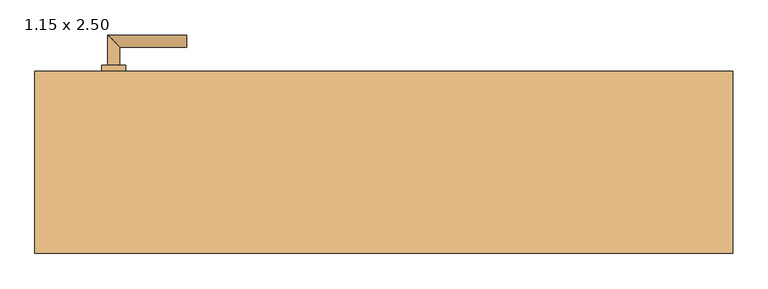
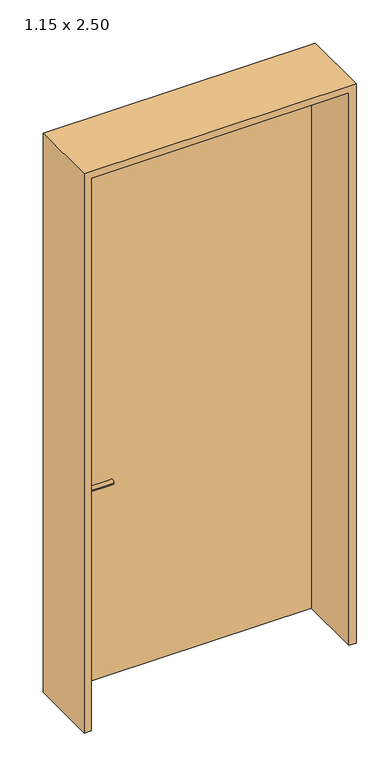
"""IFC4 building model written with IfcOpenShell, lengths in millimetres: door geometry, Drehflügel 1-flg - Blockzarge : 1.15 x 2.50."""

from ifc_helpers import new_model, si_unit, point, frame, frame_2d, origin, place, context, project, spatial, polyline, circle_curve, ellipse_curve, trimmed, segment, composite_curve, outline, extrude, source, transform, mapped, element, save
from ifc_brep_helpers import plane_surface, cylinder_surface, advanced_brep


def door_1_15_x_2_50_6bea6d7d(model_context):
    return source(origin(), model_context, "Body", "SolidModel", [
        advanced_brep(
        [(-435.0, 129.4346141, 1000.0), (-455.0, 129.4346141, 1000.0), (-435.0, 99.4346141, 1000.0), (-455.0, 79.4346141, 1000.0), (-325.0, 99.4346141, 1000.0), (-325.0, 79.4346141, 1000.0)],
        [
            (0, 1, circle_curve(frame((-445.0, 129.4346141, 1000.0), z_axis=(0.0, 1.0, 0.0), x_axis=(-1.0, 0.0, 0.0)), 10.0)),
            (1, 0, circle_curve(frame((-445.0, 129.4346141, 1000.0), z_axis=(0.0, 1.0, 0.0), x_axis=(-1.0, 0.0, 0.0)), 10.0)),
            (0, 2),
            (2, 3, ellipse_curve(frame((-445.0, 89.4346141, 1000.0), z_axis=(-0.7071067811865686, 0.7071067811865265, 0.0), x_axis=(0.7071067811865264, 0.7071067811865687, 0.0)), 14.1421356, 10.0)),
            (3, 1),
            (3, 2, ellipse_curve(frame((-445.0, 89.4346141, 1000.0), z_axis=(-0.7071067811865686, 0.7071067811865265, 0.0), x_axis=(0.7071067811865264, 0.7071067811865687, 0.0)), 14.1421356, 10.0)),
            (4, 5, circle_curve(frame((-325.0, 89.4346141, 1000.0), z_axis=(1.0, 0.0, 0.0), x_axis=(0.0, -1.0, 0.0)), 10.0)),
            (5, 4, circle_curve(frame((-325.0, 89.4346141, 1000.0), z_axis=(1.0, 0.0, 0.0), x_axis=(0.0, -1.0, 0.0)), 10.0)),
            (2, 4),
            (5, 3),
        ],
        [
            plane_surface(frame((-445.0, 129.4346141, -287.7526403), z_axis=(0.0, 1.0, 0.0), x_axis=(0.0, 0.0, 1.0))),
            cylinder_surface(frame((-445.0, 129.4346141, 1000.0), z_axis=(0.0, 1.0, 0.0), x_axis=(-1.0, 0.0, 0.0)), 10.0),
            plane_surface(frame((-325.0, 89.4346141, -287.7526403), z_axis=(1.0, 0.0, 0.0), x_axis=(0.0, 0.0, 1.0))),
            cylinder_surface(frame((-445.0, 89.4346141, 1000.0), z_axis=(-1.0, 0.0, 0.0), x_axis=(0.0, -1.0, 0.0)), 10.0),
        ],
        [
            (0, [[1, 2]]),
            (1, [[-1, 3, 4, 5]]),
            (1, [[-2, -5, 6, -3]]),
            (2, [[7, 8]]),
            (3, [[-4, 9, -8, 10]]),
            (3, [[-6, -10, -7, -9]]),
        ],
    ),
        advanced_brep(
        [(-435.0, 174.4346141, 1000.0), (-455.0, 174.4346141, 1000.0), (-435.0, 204.4346141, 1000.0), (-455.0, 224.4346141, 1000.0), (-325.0, 204.4346141, 1000.0), (-325.0, 224.4346141, 1000.0)],
        [
            (0, 1, circle_curve(frame((-445.0, 174.4346141, 1000.0), z_axis=(0.0, -1.0, 0.0), x_axis=(-1.0, 0.0, 0.0)), 10.0)),
            (1, 0, circle_curve(frame((-445.0, 174.4346141, 1000.0), z_axis=(0.0, -1.0, 0.0), x_axis=(-1.0, 0.0, 0.0)), 10.0)),
            (0, 2),
            (2, 3, ellipse_curve(frame((-445.0, 214.4346141, 1000.0), z_axis=(-0.7071067811865486, -0.7071067811865464, 0.0), x_axis=(0.7071067811865464, -0.7071067811865488, 0.0)), 14.1421356, 10.0)),
            (3, 1),
            (3, 2, ellipse_curve(frame((-445.0, 214.4346141, 1000.0), z_axis=(-0.7071067811865486, -0.7071067811865464, 0.0), x_axis=(0.7071067811865464, -0.7071067811865488, 0.0)), 14.1421356, 10.0)),
            (4, 5, circle_curve(frame((-325.0, 214.4346141, 1000.0), z_axis=(1.0, 0.0, 0.0), x_axis=(0.0, 1.0, 0.0)), 10.0)),
            (5, 4, circle_curve(frame((-325.0, 214.4346141, 1000.0), z_axis=(1.0, 0.0, 0.0), x_axis=(0.0, 1.0, 0.0)), 10.0)),
            (2, 4),
            (5, 3),
        ],
        [
            plane_surface(frame((-445.0, 174.4346141, -287.7526403), z_axis=(0.0, -1.0, 0.0), x_axis=(0.0, 0.0, 1.0))),
            cylinder_surface(frame((-445.0, 174.4346141, 1000.0), z_axis=(0.0, -1.0, 0.0), x_axis=(-1.0, 0.0, 0.0)), 10.0),
            plane_surface(frame((-325.0, 214.4346141, -287.7526403), z_axis=(1.0, 0.0, 0.0), x_axis=(0.0, 0.0, 1.0))),
            cylinder_surface(frame((-445.0, 214.4346141, 1000.0), z_axis=(-1.0, 0.0, 0.0), x_axis=(0.0, 1.0, 0.0)), 10.0),
        ],
        [
            (0, [[1, 2]]),
            (1, [[-1, 3, 4, 5]]),
            (1, [[-2, -5, 6, -3]]),
            (2, [[7, 8]]),
            (3, [[-4, 9, -8, 10]]),
            (3, [[-6, -10, -7, -9]]),
        ],
    ),
        extrude(outline(composite_curve([segment(trimmed(circle_curve(frame_2d((1000.0, -445.0)), 20.0), [point((1000.0, -425.0))], [point((1000.0, -465.0))], False, "CARTESIAN"), True, "CONTINUOUS"), segment(trimmed(circle_curve(frame_2d((1000.0, -445.0)), 20.0), [point((1000.0, -465.0))], [point((1000.0, -425.0))], False, "CARTESIAN"), True, "CONTINUOUS")], self_intersect=False)), frame((0.0, 129.4346141, 0.0), z_axis=(0.0, 1.0, 0.0), x_axis=(0.0, 0.0, 1.0)), (0.0, 0.0, 1.0), 10.0),
        extrude(outline(composite_curve([segment(trimmed(circle_curve(frame_2d((1000.0, -445.0)), 20.0), [point((1000.0, -425.0))], [point((1000.0, -465.0))], False, "CARTESIAN"), True, "CONTINUOUS"), segment(trimmed(circle_curve(frame_2d((1000.0, -445.0)), 20.0), [point((1000.0, -465.0))], [point((1000.0, -425.0))], False, "CARTESIAN"), True, "CONTINUOUS")], self_intersect=False)), frame((0.0, 164.4346141, 0.0), z_axis=(0.0, 1.0, 0.0), x_axis=(0.0, 0.0, 1.0)), (0.0, 0.0, 1.0), 10.0),
        extrude(outline(polyline([(2600.0, 575.0), (2600.0, -575.0), (100.0, -575.0), (100.0, -545.0), (2570.0, -545.0), (2570.0, 545.0), (100.0, 545.0), (100.0, 575.0), (2600.0, 575.0)])), frame((0.0, -135.5653859, 0.0), z_axis=(0.0, 1.0, 0.0), x_axis=(0.0, 0.0, 1.0)), (0.0, 0.0, 1.0), 300.0),
        extrude(outline(polyline([(545.0, 164.4346141), (545.0, 139.4346141), (-545.0, 139.4346141), (-545.0, 164.4346141), (545.0, 164.4346141)])), frame((0.0, 0.0, 100.0), z_axis=(0.0, 0.0, 1.0), x_axis=(1.0, 0.0, 0.0)), (0.0, 0.0, 1.0), 2470.0),
    ])


if __name__ == "__main__":
    model = new_model("IFC4")
    model_context = context("Model", 3, world=origin())
    ifc_project = project(units=[si_unit("LENGTHUNIT", "METRE", prefix="MILLI")], contexts=[model_context])
    site = spatial("IfcSite", under=ifc_project)
    building = spatial("IfcBuilding", under=site)
    placement = place(None, origin())
    door_1_15_x_2_50_shape = door_1_15_x_2_50_6bea6d7d(model_context)
    element("IfcDoor", 1, ObjectType="Drehflügel 1-flg - Blockzarge : 1.15 x 2.50", at=placement, inside=building, context=model_context, shape_type="MappedRepresentation", body=[
        mapped(door_1_15_x_2_50_shape, transform((0.0, 0.0, 0.0), x_axis=(1.0, 0.0, 0.0), y_axis=(0.0, 1.0, 0.0), z_axis=(0.0, 0.0, 1.0))),
    ])
    save(model, "model.ifc")

# Revit data of these elements
# Type "Drehflügel 1-flg - Blockzarge : 1.15 x 2.50"
#   Type Mark = "26"
#   Operation = "SingleSwingRight"
#   Keynote = "16.03"
#   Visual Light Transmittance = 0.9
#   Solar Heat Gain Coefficient = 0.86
#   Heat Transfer Coefficient (U) = 5.5617 W/(m²·K)
#   Rough Width = 1.150 m
#   Stärke Futter = 0.030 m
#   Rough Height [instance default] = 2.600 m
#   Höhe Türgriff = 0.900 m
#   Height = 2.500 m
#   Fußbodenaufbau [instance default] = 0.100 m
#   Width = 1.150 m
#   Sichtbarkeit Sturzlinien [instance default] = yes
#   Türgriff auswählen [instance default] = element 420047
#   Türgriff [instance default] = none
#   Türflügel [instance default] = none
#   Rahmen/Pfosten [instance default] = none
#   Construction Type Id = ""
#   Function = (empty or 0)
#   Wall Closure = (empty or 0)
#   Analytic Construction = (empty or 0)
# Element 1 (IfcDoor, "Drehflügel 1-flg - Blockzarge : 1.15 x 2.50")
#   Materials on its faces: "Metall - Chrom", "Holz - Birke"
# Materials
#   "Metall - Chrom": class "Metall", colour RGB 247 247 247, transparency 0, Cost = 0
#   "Holz - Birke": class "Holz", colour RGB 213 164 103, transparency 0, Cost = 0
